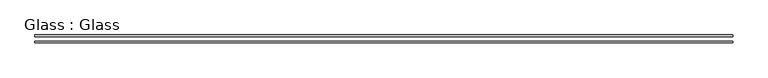
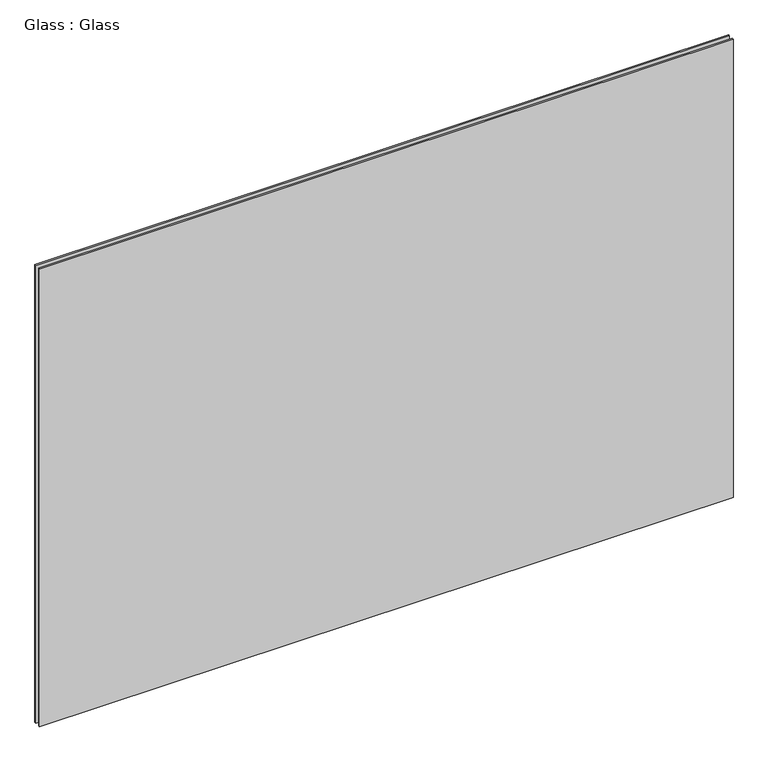
"""IFC4 building model written with IfcOpenShell, lengths in millimetres: proxy geometry, Glass : Glass."""

import ifcopenshell
import ifcopenshell.guid

model = None  # the IFC model being written
_history = None  # IfcOwnerHistory: only IFC2X3 demands one
_inside = {}  # id of a spatial element -> (the spatial element, [elements in it])
_under = {}  # id of a project, library or spatial element -> (it, [spatial elements below it])
_declared = {}  # id of a project -> (the project, [libraries it declares])
_typed = {}  # id of a type object -> (the type object, [elements of that type])
_made_of = {}  # id of a material, layer set ... -> (it, [elements and type objects made of it])


def new_model(schema):
    """Start an empty IFC model of exactly this schema.

    Asked for "IFC4X3", IfcOpenShell would pick the latest addendum, in which some entities
    have other attributes; the version numbers below select the first issue.
    IFC2X3 requires an IfcOwnerHistory on every rooted entity: one is made here for all.
    """
    global model, _history
    if schema == "IFC4X3":
        model = ifcopenshell.file(schema_version=(4, 3, 0, 0))
    else:
        model = ifcopenshell.file(schema=schema)
    _inside.clear()
    _under.clear()
    _declared.clear()
    _typed.clear()
    _made_of.clear()
    _history = None
    if model.schema == "IFC2X3":
        org = make("IfcOrganization", Name="unknown")
        user = make(
            "IfcPersonAndOrganization",
            ThePerson=make("IfcPerson", FamilyName="unknown"),
            TheOrganization=org,
        )
        app = make(
            "IfcApplication",
            ApplicationDeveloper=org,
            Version="unknown",
            ApplicationFullName="unknown",
            ApplicationIdentifier="unknown",
        )
        _history = make(
            "IfcOwnerHistory",
            OwningUser=user,
            OwningApplication=app,
            ChangeAction="ADDED",
            CreationDate=0,
        )
    return model


def make(cls, **values):
    """One entity of the class cls with the attributes given. An attribute that is None is left unset."""
    return model.create_entity(
        cls, **{name: value for name, value in values.items() if value is not None}
    )


def rooted(cls, **values):
    """An entity with a GlobalId (a new one), such as an element, a storey or a relation."""
    return make(cls, GlobalId=ifcopenshell.guid.new(), OwnerHistory=_history, **values)


def si_unit(unit_type, name, prefix=None):
    """IfcSIUnit, for example si_unit("LENGTHUNIT", "METRE", prefix="MILLI")."""
    return make("IfcSIUnit", UnitType=unit_type, Prefix=prefix, Name=name)


def assignment(units):
    """IfcUnitAssignment: the units of a project."""
    return None if units is None else make("IfcUnitAssignment", Units=units)


def point(xyz):
    """IfcCartesianPoint."""
    return None if xyz is None else make("IfcCartesianPoint", Coordinates=xyz)


def direction(xyz):
    """IfcDirection."""
    return None if xyz is None else make("IfcDirection", DirectionRatios=xyz)


def frame(location, z_axis=None, x_axis=None):
    """IfcAxis2Placement3D, a coordinate frame: its origin and axes. An axis left out is left unset."""
    return make(
        "IfcAxis2Placement3D",
        Location=point(location),
        Axis=direction(z_axis),
        RefDirection=direction(x_axis),
    )


def origin():
    """The frame at (0, 0, 0) with its axes left unset."""
    return frame((0.0, 0.0, 0.0))


def place(relative_to, where):
    """IfcLocalPlacement: puts the frame where relative to a parent placement (None: the world)."""
    return make(
        "IfcLocalPlacement", PlacementRelTo=relative_to, RelativePlacement=where
    )


def context(
    kind, dimensions, precision=None, world=None, true_north=None, identifier=None
):
    """IfcGeometricRepresentationContext, for example the 3D "Model" context."""
    return make(
        "IfcGeometricRepresentationContext",
        ContextIdentifier=identifier,
        ContextType=kind,
        CoordinateSpaceDimension=dimensions,
        Precision=precision,
        WorldCoordinateSystem=world,
        TrueNorth=true_north,
    )


def project(units=None, contexts=None):
    """IfcProject with its units and contexts."""
    return rooted(
        "IfcProject",
        Name="project",
        RepresentationContexts=contexts,
        UnitsInContext=assignment(units),
    )


def spatial(cls, under=None, at=None, **own):
    """A site, building, storey or space (cls), placed at a placement, below another one or the project."""
    s = rooted(cls, ObjectPlacement=at, **own)
    if under is not None:
        _under.setdefault(under.id(), (under, []))[1].append(s)
    return s


def polyline(points):
    """IfcPolyline through the points."""
    return make("IfcPolyline", Points=[point(p) for p in points])


def outline(outer, holes=None, kind="AREA"):
    """IfcArbitraryClosedProfileDef: a profile drawn as a closed curve; with holes, ...WithVoids."""
    if holes is None:
        return make("IfcArbitraryClosedProfileDef", ProfileType=kind, OuterCurve=outer)
    return make(
        "IfcArbitraryProfileDefWithVoids",
        ProfileType=kind,
        OuterCurve=outer,
        InnerCurves=holes,
    )


def extrude(swept, where, along, depth):
    """IfcExtrudedAreaSolid: the profile swept, set in the frame where, extruded along a direction by depth."""
    return make(
        "IfcExtrudedAreaSolid",
        SweptArea=swept,
        Position=where,
        ExtrudedDirection=direction(along),
        Depth=depth,
    )


def shape(context_of_items, identifier, shape_type, items):
    """IfcShapeRepresentation: the items that make up one representation, for example the "Body"."""
    return make(
        "IfcShapeRepresentation",
        ContextOfItems=context_of_items,
        RepresentationIdentifier=identifier,
        RepresentationType=shape_type,
        Items=items,
    )


def source(mapping_origin, context_of_items, identifier, shape_type, items):
    """IfcRepresentationMap: a shape defined once, which mapped items show again and again."""
    return make(
        "IfcRepresentationMap",
        MappingOrigin=mapping_origin,
        MappedRepresentation=shape(context_of_items, identifier, shape_type, items),
    )


def transform(
    local_origin,
    x_axis=None,
    y_axis=None,
    z_axis=None,
    scale=None,
    scale2=None,
    scale3=None,
    uniform=True,
):
    """IfcCartesianTransformationOperator3D, or its non-uniform kind. x_axis, y_axis, z_axis: its Axis1, 2, 3."""
    if uniform:
        return make(
            "IfcCartesianTransformationOperator3D",
            Axis1=direction(x_axis),
            Axis2=direction(y_axis),
            LocalOrigin=point(local_origin),
            Scale=scale,
            Axis3=direction(z_axis),
        )
    return make(
        "IfcCartesianTransformationOperator3DnonUniform",
        Axis1=direction(x_axis),
        Axis2=direction(y_axis),
        LocalOrigin=point(local_origin),
        Scale=scale,
        Axis3=direction(z_axis),
        Scale2=scale2,
        Scale3=scale3,
    )


def mapped(mapping_source, mapping_target):
    """IfcMappedItem: shows the shape of a source again, moved by a transform."""
    return make(
        "IfcMappedItem", MappingSource=mapping_source, MappingTarget=mapping_target
    )


def made_of(thing, what):
    """Note that an element or type object is made of a material, layer set ...; save() writes the relation."""
    if what is not None:
        _made_of.setdefault(what.id(), (what, []))[1].append(thing)
    return thing


def element(
    cls,
    number,
    at=None,
    inside=None,
    cuts=None,
    type_object=None,
    material=None,
    context=None,
    identifier="Body",
    shape_type=None,
    held_by="IfcProductDefinitionShape",
    body=None,
    shapes=None,
    **own,
):
    """One element of the class cls, such as IfcWall. Its Tag is "e" and its number.

    at: its placement. inside: the storey or other place that contains it. cuts: it is an
    opening in that element (IfcRelVoidsElement). A single representation is given by context,
    identifier, shape_type and body (its items); several are given by shapes. held_by: the class
    of the entity that holds the representations. save() writes the other relations.
    """
    e = rooted(cls, Tag="e%d" % number, ObjectPlacement=at, **own)
    if body is not None:
        shapes = [shape(context, identifier, shape_type, body)]
    if shapes is not None:
        e.Representation = make(held_by, Representations=shapes)
    if inside is not None:
        _inside.setdefault(inside.id(), (inside, []))[1].append(e)
    if cuts is not None:
        rooted(
            "IfcRelVoidsElement", RelatingBuildingElement=cuts, RelatedOpeningElement=e
        )
    if type_object is not None:
        _typed.setdefault(type_object.id(), (type_object, []))[1].append(e)
    return made_of(e, material)


def aggregate(whole, parts):
    """IfcRelAggregates: a whole, such as a stair, and the parts it consists of."""
    return rooted("IfcRelAggregates", RelatingObject=whole, RelatedObjects=parts)


def save(model, path):
    """Write the relations noted so far, then the file.

    IfcRelAggregates (storeys below a building ...), IfcRelContainedInSpatialStructure (elements
    in a storey), IfcRelDefinesByType, IfcRelAssociatesMaterial and IfcRelDeclares: one each for
    every whole, place, type object, material and project.
    """
    for whole, parts in _under.values():
        aggregate(whole, parts)
    for where, things in _inside.values():
        rooted(
            "IfcRelContainedInSpatialStructure",
            RelatedElements=things,
            RelatingStructure=where,
        )
    for kind, things in _typed.values():
        rooted("IfcRelDefinesByType", RelatedObjects=things, RelatingType=kind)
    for what, things in _made_of.values():
        rooted("IfcRelAssociatesMaterial", RelatedObjects=things, RelatingMaterial=what)
    for by, libraries in _declared.values():
        rooted("IfcRelDeclares", RelatingContext=by, RelatedDefinitions=libraries)
    model.write(path)


def glass_glass_7f8999f5(model_context):
    return source(origin(), model_context, "Body", "SweptSolid", [
        extrude(outline(polyline([(14383.0178845, -4394.1834255), (14383.0178845, -4398.9459255), (12383.0178845, -4398.9459255), (12383.0178845, -4394.1834255), (14383.0178845, -4394.1834255)])), frame((0.0, 0.0, 41130.5392812), z_axis=(0.0, 0.0, 1.0), x_axis=(1.0, 0.0, 0.0)), (0.0, 0.0, 1.0), 1396.8024401),
        extrude(outline(polyline([(14383.0178845, -4412.1834255), (14383.0178845, -4416.9459255), (12383.0178845, -4416.9459255), (12383.0178845, -4412.1834255), (14383.0178845, -4412.1834255)])), frame((0.0, 0.0, 41130.5392812), z_axis=(0.0, 0.0, 1.0), x_axis=(1.0, 0.0, 0.0)), (0.0, 0.0, 1.0), 1396.8024401),
    ])


if __name__ == "__main__":
    model = new_model("IFC4")
    model_context = context("Model", 3, world=origin())
    ifc_project = project(units=[si_unit("LENGTHUNIT", "METRE", prefix="MILLI")], contexts=[model_context])
    site = spatial("IfcSite", under=ifc_project)
    building = spatial("IfcBuilding", under=site)
    placement = place(None, origin())
    glass_glass_shape = glass_glass_7f8999f5(model_context)
    element("IfcBuildingElementProxy", 1, Name="Glass : Glass", ObjectType="Glass : Glass", at=placement, inside=building, context=model_context, shape_type="MappedRepresentation", body=[
        mapped(glass_glass_shape, transform((0.0, 0.0, 0.0), x_axis=(1.0, 0.0, 0.0), y_axis=(0.0, 1.0, 0.0), z_axis=(0.0, 0.0, 1.0))),
    ])
    save(model, "model.ifc")

# Revit data of these elements
# Type "Glass : Glass"
#   NameOverride = "Glass"
# Element 1 (IfcBuildingElementProxy, "Glass : Glass")
#   Materials on its faces: "1\" INSULATED GLAZING"
# Materials
#   "1\" INSULATED GLAZING": class "Unassigned", colour RGB 146 199 212, transparency 0
